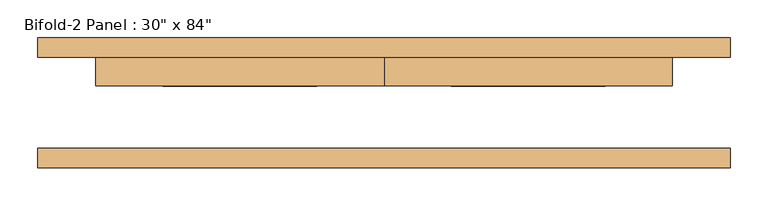
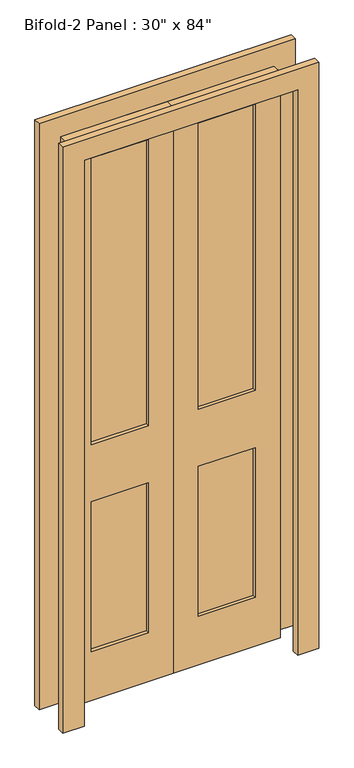
"""IFC4 building model written with IfcOpenShell, lengths in millimetres: door geometry."""

from ifc_helpers import new_model, si_unit, frame, origin, place, context, project, spatial, polyline, outline, extrude, source, transform, mapped, element, save


def door_ba29ed12(model_context):
    return source(origin(), model_context, "Body", "SweptSolid", [
        extrude(outline(polyline([(2133.6, 0.0), (2133.6, -381.0), (0.0, -381.0), (0.0, 0.0), (2133.6, 0.0)]), holes=[polyline([(2044.7, -88.9), (965.11872, -88.9), (965.11872, -292.1), (2044.7, -292.1), (2044.7, -88.9)]), polyline([(749.3, -88.9), (184.15, -88.9), (184.15, -292.1), (749.3, -292.1), (749.3, -88.9)])]), frame((0.0, 22.225, 0.0), z_axis=(0.0, 1.0, 0.0), x_axis=(0.0, 0.0, 1.0)), (0.0, 0.0, 1.0), 38.1),
        extrude(outline(polyline([(-88.9, 34.925), (-292.1, 34.925), (-292.1, 47.625), (-88.9, 47.625), (-88.9, 34.925)])), frame((0.0, 0.0, 965.11872), z_axis=(0.0, 0.0, 1.0), x_axis=(1.0, 0.0, 0.0)), (0.0, 0.0, 1.0), 1079.58128),
        extrude(outline(polyline([(-88.9, 34.925), (-292.1, 34.925), (-292.1, 47.625), (-88.9, 47.625), (-88.9, 34.925)])), frame((0.0, 0.0, 184.15), z_axis=(0.0, 0.0, 1.0), x_axis=(1.0, 0.0, 0.0)), (0.0, 0.0, 1.0), 565.15),
        extrude(outline(polyline([(292.1, 34.925), (88.9, 34.925), (88.9, 47.625), (292.1, 47.625), (292.1, 34.925)])), frame((0.0, 0.0, 965.11872), z_axis=(0.0, 0.0, 1.0), x_axis=(1.0, 0.0, 0.0)), (0.0, 0.0, 1.0), 1079.58128),
        extrude(outline(polyline([(292.1, 34.925), (88.9, 34.925), (88.9, 47.625), (292.1, 47.625), (292.1, 34.925)])), frame((0.0, 0.0, 184.15), z_axis=(0.0, 0.0, 1.0), x_axis=(1.0, 0.0, 0.0)), (0.0, 0.0, 1.0), 565.15),
        extrude(outline(polyline([(2209.8, -457.2), (0.0, -457.2), (0.0, -381.0), (2133.6, -381.0), (2133.6, 381.0), (0.0, 381.0), (0.0, 457.2), (2209.8, 457.2), (2209.8, -457.2)])), frame((0.0, 60.325, 0.0), z_axis=(0.0, 1.0, 0.0), x_axis=(0.0, 0.0, 1.0)), (0.0, 0.0, 1.0), 25.4),
        extrude(outline(polyline([(2209.8, 457.2), (2209.8, -457.2), (0.0, -457.2), (0.0, -381.0), (2133.6, -381.0), (2133.6, 381.0), (0.0, 381.0), (0.0, 457.2), (2209.8, 457.2)])), frame((0.0, -85.725, 0.0), z_axis=(0.0, 1.0, 0.0), x_axis=(0.0, 0.0, 1.0)), (0.0, 0.0, 1.0), 25.4),
        extrude(outline(polyline([(2133.6, 381.0), (2133.6, 0.0), (0.0, 0.0), (0.0, 381.0), (2133.6, 381.0)]), holes=[polyline([(2044.7, 88.9), (2044.7, 292.1), (965.11872, 292.1), (965.11872, 88.9), (2044.7, 88.9)]), polyline([(749.3, 88.9), (749.3, 292.1), (184.15, 292.1), (184.15, 88.9), (749.3, 88.9)])]), frame((0.0, 22.225, 0.0), z_axis=(0.0, 1.0, 0.0), x_axis=(0.0, 0.0, 1.0)), (0.0, 0.0, 1.0), 38.1),
    ])


if __name__ == "__main__":
    model = new_model("IFC4")
    model_context = context("Model", 3, world=origin())
    ifc_project = project(units=[si_unit("LENGTHUNIT", "METRE", prefix="MILLI")], contexts=[model_context])
    site = spatial("IfcSite", under=ifc_project)
    building = spatial("IfcBuilding", under=site)
    placement = place(None, origin())
    door_shape = door_ba29ed12(model_context)
    element("IfcDoor", 1, ObjectType="Bifold-2 Panel : 30\" x 84\"", at=placement, inside=building, context=model_context, shape_type="MappedRepresentation", body=[
        mapped(door_shape, transform((0.0, 0.0, 0.0), x_axis=(1.0, 0.0, 0.0), y_axis=(0.0, 1.0, 0.0), z_axis=(0.0, 0.0, 1.0))),
    ])
    save(model, "model.ifc")

# Revit data of these elements
# Type "Bifold-2 Panel : 30\" x 84\""
#   Type Mark = "35"
#   Assembly Code = "C1020"
#   Thickness = 0' - 1 1/2"
#   Height = 7' - 0"
#   Trim Projection Ext = 0' - 1"
#   Trim Projection Int = 0' - 1"
#   Trim Width = 0' - 3"
#   Width = 2' - 6"
#   Door Material = Door - Panel
#   Frame Material = Door - Frame
#   Function = (empty or 0)
#   Wall Closure = (empty or 0)
# Element 1 (IfcDoor, "Bifold-2 Panel : 30\" x 84\"")
#   Materials on its faces: "Door - Panel", "Door - Frame"
# Materials
#   "Door - Panel": class "Wood", colour RGB 210 159 95, transparency 0, Cost = 0
#   "Door - Frame": class "Miscellaneous", colour RGB 118 70 51, transparency 0, Cost = 0
